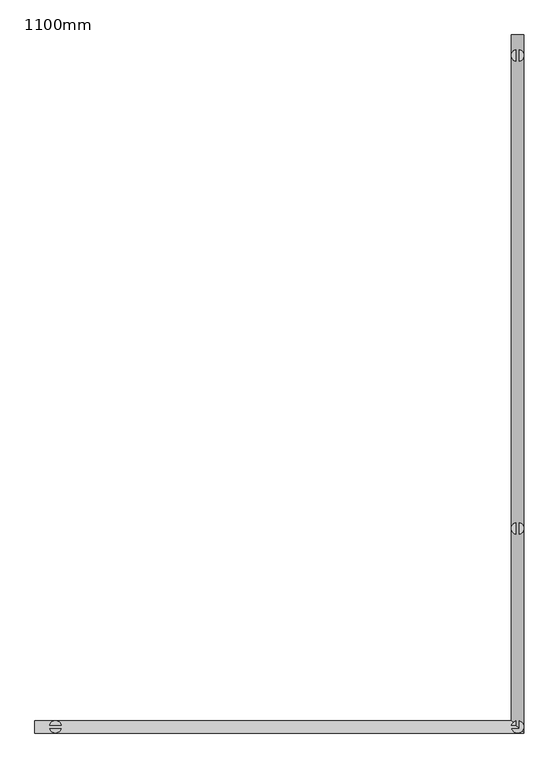
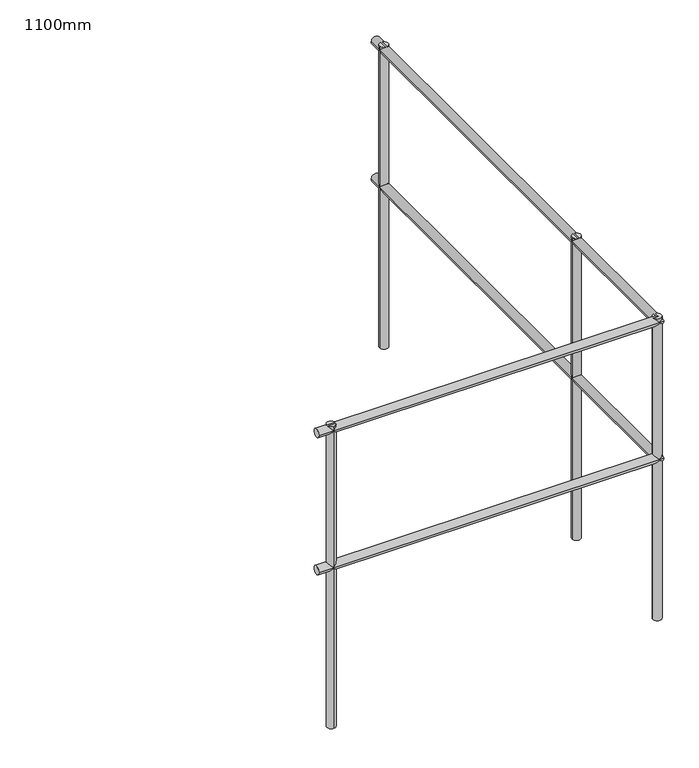
"""IFC4 building model written with IfcOpenShell, lengths in millimetres: railing geometry, 1100mm."""

import ifcopenshell
import ifcopenshell.guid

model = None  # the IFC model being written
_history = None  # IfcOwnerHistory: only IFC2X3 demands one
_inside = {}  # id of a spatial element -> (the spatial element, [elements in it])
_under = {}  # id of a project, library or spatial element -> (it, [spatial elements below it])
_declared = {}  # id of a project -> (the project, [libraries it declares])
_typed = {}  # id of a type object -> (the type object, [elements of that type])
_made_of = {}  # id of a material, layer set ... -> (it, [elements and type objects made of it])


def new_model(schema):
    """Start an empty IFC model of exactly this schema.

    Asked for "IFC4X3", IfcOpenShell would pick the latest addendum, in which some entities
    have other attributes; the version numbers below select the first issue.
    IFC2X3 requires an IfcOwnerHistory on every rooted entity: one is made here for all.
    """
    global model, _history
    if schema == "IFC4X3":
        model = ifcopenshell.file(schema_version=(4, 3, 0, 0))
    else:
        model = ifcopenshell.file(schema=schema)
    _inside.clear()
    _under.clear()
    _declared.clear()
    _typed.clear()
    _made_of.clear()
    _history = None
    if model.schema == "IFC2X3":
        org = make("IfcOrganization", Name="unknown")
        user = make(
            "IfcPersonAndOrganization",
            ThePerson=make("IfcPerson", FamilyName="unknown"),
            TheOrganization=org,
        )
        app = make(
            "IfcApplication",
            ApplicationDeveloper=org,
            Version="unknown",
            ApplicationFullName="unknown",
            ApplicationIdentifier="unknown",
        )
        _history = make(
            "IfcOwnerHistory",
            OwningUser=user,
            OwningApplication=app,
            ChangeAction="ADDED",
            CreationDate=0,
        )
    return model


def make(cls, **values):
    """One entity of the class cls with the attributes given. An attribute that is None is left unset."""
    return model.create_entity(
        cls, **{name: value for name, value in values.items() if value is not None}
    )


def rooted(cls, **values):
    """An entity with a GlobalId (a new one), such as an element, a storey or a relation."""
    return make(cls, GlobalId=ifcopenshell.guid.new(), OwnerHistory=_history, **values)


def si_unit(unit_type, name, prefix=None):
    """IfcSIUnit, for example si_unit("LENGTHUNIT", "METRE", prefix="MILLI")."""
    return make("IfcSIUnit", UnitType=unit_type, Prefix=prefix, Name=name)


def assignment(units):
    """IfcUnitAssignment: the units of a project."""
    return None if units is None else make("IfcUnitAssignment", Units=units)


def point(xyz):
    """IfcCartesianPoint."""
    return None if xyz is None else make("IfcCartesianPoint", Coordinates=xyz)


def direction(xyz):
    """IfcDirection."""
    return None if xyz is None else make("IfcDirection", DirectionRatios=xyz)


def frame(location, z_axis=None, x_axis=None):
    """IfcAxis2Placement3D, a coordinate frame: its origin and axes. An axis left out is left unset."""
    return make(
        "IfcAxis2Placement3D",
        Location=point(location),
        Axis=direction(z_axis),
        RefDirection=direction(x_axis),
    )


def frame_2d(location, x_axis=None):
    """IfcAxis2Placement2D, a coordinate frame in the plane: its origin and x axis."""
    return make(
        "IfcAxis2Placement2D", Location=point(location), RefDirection=direction(x_axis)
    )


def origin():
    """The frame at (0, 0, 0) with its axes left unset."""
    return frame((0.0, 0.0, 0.0))


def place(relative_to, where):
    """IfcLocalPlacement: puts the frame where relative to a parent placement (None: the world)."""
    return make(
        "IfcLocalPlacement", PlacementRelTo=relative_to, RelativePlacement=where
    )


def context(
    kind, dimensions, precision=None, world=None, true_north=None, identifier=None
):
    """IfcGeometricRepresentationContext, for example the 3D "Model" context."""
    return make(
        "IfcGeometricRepresentationContext",
        ContextIdentifier=identifier,
        ContextType=kind,
        CoordinateSpaceDimension=dimensions,
        Precision=precision,
        WorldCoordinateSystem=world,
        TrueNorth=true_north,
    )


def project(units=None, contexts=None):
    """IfcProject with its units and contexts."""
    return rooted(
        "IfcProject",
        Name="project",
        RepresentationContexts=contexts,
        UnitsInContext=assignment(units),
    )


def spatial(cls, under=None, at=None, **own):
    """A site, building, storey or space (cls), placed at a placement, below another one or the project."""
    s = rooted(cls, ObjectPlacement=at, **own)
    if under is not None:
        _under.setdefault(under.id(), (under, []))[1].append(s)
    return s


def circle_curve(where, radius):
    """IfcCircle in the frame where."""
    return make("IfcCircle", Position=where, Radius=radius)


def ellipse_curve(where, semi_axis1, semi_axis2):
    """IfcEllipse in the frame where."""
    return make(
        "IfcEllipse", Position=where, SemiAxis1=semi_axis1, SemiAxis2=semi_axis2
    )


def trimmed(basis, trim1, trim2, sense, master):
    """IfcTrimmedCurve: the piece of a basis curve between two trims."""
    return make(
        "IfcTrimmedCurve",
        BasisCurve=basis,
        Trim1=trim1,
        Trim2=trim2,
        SenseAgreement=sense,
        MasterRepresentation=master,
    )


def segment(curve, same_sense, transition):
    """IfcCompositeCurveSegment."""
    return make(
        "IfcCompositeCurveSegment",
        Transition=transition,
        SameSense=same_sense,
        ParentCurve=curve,
    )


def composite_curve(segments, self_intersect=None):
    """IfcCompositeCurve: segments joined end to end."""
    return make("IfcCompositeCurve", Segments=segments, SelfIntersect=self_intersect)


def outline(outer, holes=None, kind="AREA"):
    """IfcArbitraryClosedProfileDef: a profile drawn as a closed curve; with holes, ...WithVoids."""
    if holes is None:
        return make("IfcArbitraryClosedProfileDef", ProfileType=kind, OuterCurve=outer)
    return make(
        "IfcArbitraryProfileDefWithVoids",
        ProfileType=kind,
        OuterCurve=outer,
        InnerCurves=holes,
    )


def extrude(swept, where, along, depth):
    """IfcExtrudedAreaSolid: the profile swept, set in the frame where, extruded along a direction by depth."""
    return make(
        "IfcExtrudedAreaSolid",
        SweptArea=swept,
        Position=where,
        ExtrudedDirection=direction(along),
        Depth=depth,
    )


def shape(context_of_items, identifier, shape_type, items):
    """IfcShapeRepresentation: the items that make up one representation, for example the "Body"."""
    return make(
        "IfcShapeRepresentation",
        ContextOfItems=context_of_items,
        RepresentationIdentifier=identifier,
        RepresentationType=shape_type,
        Items=items,
    )


def source(mapping_origin, context_of_items, identifier, shape_type, items):
    """IfcRepresentationMap: a shape defined once, which mapped items show again and again."""
    return make(
        "IfcRepresentationMap",
        MappingOrigin=mapping_origin,
        MappedRepresentation=shape(context_of_items, identifier, shape_type, items),
    )


def transform(
    local_origin,
    x_axis=None,
    y_axis=None,
    z_axis=None,
    scale=None,
    scale2=None,
    scale3=None,
    uniform=True,
):
    """IfcCartesianTransformationOperator3D, or its non-uniform kind. x_axis, y_axis, z_axis: its Axis1, 2, 3."""
    if uniform:
        return make(
            "IfcCartesianTransformationOperator3D",
            Axis1=direction(x_axis),
            Axis2=direction(y_axis),
            LocalOrigin=point(local_origin),
            Scale=scale,
            Axis3=direction(z_axis),
        )
    return make(
        "IfcCartesianTransformationOperator3DnonUniform",
        Axis1=direction(x_axis),
        Axis2=direction(y_axis),
        LocalOrigin=point(local_origin),
        Scale=scale,
        Axis3=direction(z_axis),
        Scale2=scale2,
        Scale3=scale3,
    )


def mapped(mapping_source, mapping_target):
    """IfcMappedItem: shows the shape of a source again, moved by a transform."""
    return make(
        "IfcMappedItem", MappingSource=mapping_source, MappingTarget=mapping_target
    )


def made_of(thing, what):
    """Note that an element or type object is made of a material, layer set ...; save() writes the relation."""
    if what is not None:
        _made_of.setdefault(what.id(), (what, []))[1].append(thing)
    return thing


def element(
    cls,
    number,
    at=None,
    inside=None,
    cuts=None,
    type_object=None,
    material=None,
    context=None,
    identifier="Body",
    shape_type=None,
    held_by="IfcProductDefinitionShape",
    body=None,
    shapes=None,
    **own,
):
    """One element of the class cls, such as IfcWall. Its Tag is "e" and its number.

    at: its placement. inside: the storey or other place that contains it. cuts: it is an
    opening in that element (IfcRelVoidsElement). A single representation is given by context,
    identifier, shape_type and body (its items); several are given by shapes. held_by: the class
    of the entity that holds the representations. save() writes the other relations.
    """
    e = rooted(cls, Tag="e%d" % number, ObjectPlacement=at, **own)
    if body is not None:
        shapes = [shape(context, identifier, shape_type, body)]
    if shapes is not None:
        e.Representation = make(held_by, Representations=shapes)
    if inside is not None:
        _inside.setdefault(inside.id(), (inside, []))[1].append(e)
    if cuts is not None:
        rooted(
            "IfcRelVoidsElement", RelatingBuildingElement=cuts, RelatedOpeningElement=e
        )
    if type_object is not None:
        _typed.setdefault(type_object.id(), (type_object, []))[1].append(e)
    return made_of(e, material)


def aggregate(whole, parts):
    """IfcRelAggregates: a whole, such as a stair, and the parts it consists of."""
    return rooted("IfcRelAggregates", RelatingObject=whole, RelatedObjects=parts)


def save(model, path):
    """Write the relations noted so far, then the file.

    IfcRelAggregates (storeys below a building ...), IfcRelContainedInSpatialStructure (elements
    in a storey), IfcRelDefinesByType, IfcRelAssociatesMaterial and IfcRelDeclares: one each for
    every whole, place, type object, material and project.
    """
    for whole, parts in _under.values():
        aggregate(whole, parts)
    for where, things in _inside.values():
        rooted(
            "IfcRelContainedInSpatialStructure",
            RelatedElements=things,
            RelatingStructure=where,
        )
    for kind, things in _typed.values():
        rooted("IfcRelDefinesByType", RelatedObjects=things, RelatingType=kind)
    for what, things in _made_of.values():
        rooted("IfcRelAssociatesMaterial", RelatedObjects=things, RelatingMaterial=what)
    for by, libraries in _declared.values():
        rooted("IfcRelDeclares", RelatingContext=by, RelatedDefinitions=libraries)
    model.write(path)


def plane_surface(at):
    """IfcPlane: the flat surface through the origin of the frame at, square to its z axis."""
    return make("IfcPlane", Position=at)


def cylinder_surface(at, radius):
    """IfcCylindricalSurface: all points at the distance radius from the z axis of the frame at."""
    return make("IfcCylindricalSurface", Position=at, Radius=radius)


def advanced_brep(points, edges, surfaces, faces):
    """IfcAdvancedBrep: a solid bounded by faces that lie on surfaces and meet in shared edges.

    An edge is (start, end): straight between two places in points (the first is 0);
    or (start, end, curve); or (start, end, curve, False) where it runs against its curve.
    A face is (place in surfaces, loops), or (place, loops, False) where it looks against
    its surface's normal. A loop lists edges by number (the first is 1), with a minus sign
    where the edge is run from its end to its start. The first loop is the outer one.
    """
    corners = [point(p) for p in points]
    vertices = [make("IfcVertexPoint", VertexGeometry=c) for c in corners]
    made = []
    for start, end, *more in edges:
        made.append(
            make(
                "IfcEdgeCurve",
                EdgeStart=vertices[start],
                EdgeEnd=vertices[end],
                EdgeGeometry=more[0] if more else make("IfcPolyline", Points=[corners[start], corners[end]]),
                SameSense=more[1] if len(more) > 1 else True,
            )
        )
    hull = []
    for where, loops, *sense in faces:
        bounds = []
        for j, loop in enumerate(loops):
            ring = [make("IfcOrientedEdge", EdgeElement=made[abs(k) - 1], Orientation=k > 0) for k in loop]
            bounds.append(
                make(
                    "IfcFaceOuterBound" if j == 0 else "IfcFaceBound",
                    Bound=make("IfcEdgeLoop", EdgeList=ring),
                    Orientation=True,
                )
            )
        hull.append(make("IfcAdvancedFace", Bounds=bounds, FaceSurface=surfaces[where], SameSense=sense[0] if sense else True))
    return make("IfcAdvancedBrep", Outer=make("IfcClosedShell", CfsFaces=hull))


def railing_1100mm_da86e9fc(model_context):
    return source(origin(), model_context, "Body", "SolidModel", [
        advanced_brep(
        [(11414.7052251, 14979.5208589, 4745.0), (11384.7052251, 14979.5208589, 4745.0), (10225.0, 13282.0208589, 4745.0), (10225.0, 13312.0208589, 4745.0), (11414.7052251, 13282.0208589, 4745.0), (11384.7052251, 13312.0208589, 4745.0)],
        [
            (0, 1, circle_curve(frame((11399.7052251, 14979.5208589, 4745.0), z_axis=(0.0, 1.0, 0.0), x_axis=(-1.0, 0.0, 0.0)), 15.0)),
            (1, 0, circle_curve(frame((11399.7052251, 14979.5208589, 4745.0), z_axis=(0.0, 1.0, 0.0), x_axis=(-1.0, 0.0, 0.0)), 15.0)),
            (2, 3, circle_curve(frame((10225.0, 13297.0208589, 4745.0), z_axis=(-1.0, 0.0, 0.0), x_axis=(0.0, 1.0, 0.0)), 15.0)),
            (3, 2, circle_curve(frame((10225.0, 13297.0208589, 4745.0), z_axis=(-1.0, 0.0, 0.0), x_axis=(0.0, 1.0, 0.0)), 15.0)),
            (0, 4),
            (4, 5, ellipse_curve(frame((11399.7052251, 13297.0208589, 4745.0), z_axis=(0.7071067811865493, 0.7071067811865457, 0.0), x_axis=(-0.7071067811865457, 0.7071067811865493, 0.0)), 21.2132034, 15.0)),
            (5, 1),
            (5, 4, ellipse_curve(frame((11399.7052251, 13297.0208589, 4745.0), z_axis=(0.7071067811865493, 0.7071067811865457, 0.0), x_axis=(-0.7071067811865457, 0.7071067811865493, 0.0)), 21.2132034, 15.0)),
            (4, 2),
            (3, 5),
        ],
        [
            plane_surface(frame((11399.7052251, 14979.5208589, 4760.0), z_axis=(0.0, 1.0, 0.0), x_axis=(0.0, 0.0, -1.0))),
            plane_surface(frame((10225.0, 13297.0208589, 4760.0), z_axis=(-1.0, 0.0, 0.0), x_axis=(0.0, -1.0, 0.0))),
            cylinder_surface(frame((11399.7052251, 14979.5208589, 4745.0), z_axis=(0.0, 1.0, 0.0), x_axis=(-1.0, 0.0, 0.0)), 15.0),
            cylinder_surface(frame((11399.7052251, 13297.0208589, 4745.0), z_axis=(1.0, 0.0, 0.0), x_axis=(0.0, 1.0, 0.0)), 15.0),
        ],
        [
            (0, [[1, 2]]),
            (1, [[3, 4]]),
            (2, [[-1, 5, 6, 7]]),
            (2, [[-2, -7, 8, -5]]),
            (3, [[-6, 9, -4, 10]]),
            (3, [[-8, -10, -3, -9]]),
        ],
    ),
        advanced_brep(
        [(11414.7052251, 14979.5208589, 5245.0), (11384.7052251, 14979.5208589, 5245.0), (11414.7052251, 13282.0208589, 5245.0), (11384.7052251, 13312.0208589, 5245.0), (10225.0, 13282.0208589, 5245.0), (10225.0, 13312.0208589, 5245.0)],
        [
            (0, 1, circle_curve(frame((11399.7052251, 14979.5208589, 5245.0), z_axis=(0.0, 1.0, 0.0), x_axis=(-1.0, 0.0, 0.0)), 15.0)),
            (1, 0, circle_curve(frame((11399.7052251, 14979.5208589, 5245.0), z_axis=(0.0, 1.0, 0.0), x_axis=(-1.0, 0.0, 0.0)), 15.0)),
            (0, 2),
            (2, 3, ellipse_curve(frame((11399.7052251, 13297.0208589, 5245.0), z_axis=(0.7071067811865493, 0.7071067811865457, 0.0), x_axis=(-0.7071067811865457, 0.7071067811865493, 0.0)), 21.2132034, 15.0)),
            (3, 1),
            (3, 2, ellipse_curve(frame((11399.7052251, 13297.0208589, 5245.0), z_axis=(0.7071067811865493, 0.7071067811865457, 0.0), x_axis=(-0.7071067811865457, 0.7071067811865493, 0.0)), 21.2132034, 15.0)),
            (4, 5, circle_curve(frame((10225.0, 13297.0208589, 5245.0), z_axis=(-1.0, 0.0, 0.0), x_axis=(0.0, 1.0, 0.0)), 15.0)),
            (5, 4, circle_curve(frame((10225.0, 13297.0208589, 5245.0), z_axis=(-1.0, 0.0, 0.0), x_axis=(0.0, 1.0, 0.0)), 15.0)),
            (2, 4),
            (5, 3),
        ],
        [
            plane_surface(frame((11399.7052251, 14979.5208589, 5260.0), z_axis=(0.0, 1.0, 0.0), x_axis=(0.0, 0.0, -1.0))),
            cylinder_surface(frame((11399.7052251, 14979.5208589, 5245.0), z_axis=(0.0, 1.0, 0.0), x_axis=(-1.0, 0.0, 0.0)), 15.0),
            plane_surface(frame((10225.0, 13297.0208589, 5260.0), z_axis=(-1.0, 0.0, 0.0), x_axis=(0.0, -1.0, 0.0))),
            cylinder_surface(frame((11399.7052251, 13297.0208589, 5245.0), z_axis=(1.0, 0.0, 0.0), x_axis=(0.0, 1.0, 0.0)), 15.0),
        ],
        [
            (0, [[1, 2]]),
            (1, [[-1, 3, 4, 5]]),
            (1, [[-2, -5, 6, -3]]),
            (2, [[7, 8]]),
            (3, [[-4, 9, -8, 10]]),
            (3, [[-6, -10, -7, -9]]),
        ],
    ),
        extrude(outline(composite_curve([segment(trimmed(circle_curve(frame_2d((11399.7052251, 13779.5208589)), 15.0), [point((11384.7052251, 13779.5208589))], [point((11414.7052251, 13779.5208589))], False, "CARTESIAN"), True, "CONTINUOUS"), segment(trimmed(circle_curve(frame_2d((11399.7052251, 13779.5208589)), 15.0), [point((11414.7052251, 13779.5208589))], [point((11384.7052251, 13779.5208589))], False, "CARTESIAN"), True, "CONTINUOUS")], self_intersect=False)), frame((0.0, 0.0, 4160.0), z_axis=(0.0, 0.0, 1.0), x_axis=(1.0, 0.0, 0.0)), (0.0, 0.0, 1.0), 1100.0),
        extrude(outline(composite_curve([segment(trimmed(circle_curve(frame_2d((11399.7052251, 13297.0208589)), 15.0), [point((11384.7052251, 13297.0208589))], [point((11414.7052251, 13297.0208589))], False, "CARTESIAN"), True, "CONTINUOUS"), segment(trimmed(circle_curve(frame_2d((11399.7052251, 13297.0208589)), 15.0), [point((11414.7052251, 13297.0208589))], [point((11384.7052251, 13297.0208589))], False, "CARTESIAN"), True, "CONTINUOUS")], self_intersect=False)), frame((0.0, 0.0, 4160.0), z_axis=(0.0, 0.0, 1.0), x_axis=(1.0, 0.0, 0.0)), (0.0, 0.0, 1.0), 1100.0),
        extrude(outline(composite_curve([segment(trimmed(circle_curve(frame_2d((10275.0, 13297.0208589)), 15.0), [point((10275.0, 13312.0208589))], [point((10275.0, 13282.0208589))], False, "CARTESIAN"), True, "CONTINUOUS"), segment(trimmed(circle_curve(frame_2d((10275.0, 13297.0208589)), 15.0), [point((10275.0, 13282.0208589))], [point((10275.0, 13312.0208589))], False, "CARTESIAN"), True, "CONTINUOUS")], self_intersect=False)), frame((0.0, 0.0, 4160.0), z_axis=(0.0, 0.0, 1.0), x_axis=(1.0, 0.0, 0.0)), (0.0, 0.0, 1.0), 1100.0),
        extrude(outline(composite_curve([segment(trimmed(circle_curve(frame_2d((11399.7052251, 14929.5208589)), 15.0), [point((11384.7052251, 14929.5208589))], [point((11414.7052251, 14929.5208589))], False, "CARTESIAN"), True, "CONTINUOUS"), segment(trimmed(circle_curve(frame_2d((11399.7052251, 14929.5208589)), 15.0), [point((11414.7052251, 14929.5208589))], [point((11384.7052251, 14929.5208589))], False, "CARTESIAN"), True, "CONTINUOUS")], self_intersect=False)), frame((0.0, 0.0, 4160.0), z_axis=(0.0, 0.0, 1.0), x_axis=(1.0, 0.0, 0.0)), (0.0, 0.0, 1.0), 1100.0),
    ])


if __name__ == "__main__":
    model = new_model("IFC4")
    model_context = context("Model", 3, world=origin())
    ifc_project = project(units=[si_unit("LENGTHUNIT", "METRE", prefix="MILLI")], contexts=[model_context])
    site = spatial("IfcSite", under=ifc_project)
    building = spatial("IfcBuilding", under=site)
    placement = place(None, origin())
    railing_1100mm_shape = railing_1100mm_da86e9fc(model_context)
    element("IfcRailing", 1, ObjectType="1100mm", at=placement, inside=building, context=model_context, shape_type="MappedRepresentation", body=[
        mapped(railing_1100mm_shape, transform((0.0, 0.0, 0.0), x_axis=(1.0, 0.0, 0.0), y_axis=(0.0, 1.0, 0.0), z_axis=(0.0, 0.0, 1.0))),
    ])
    save(model, "model.ifc")
